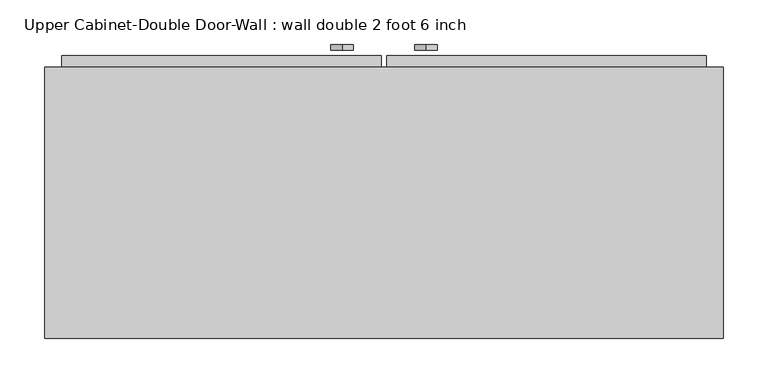
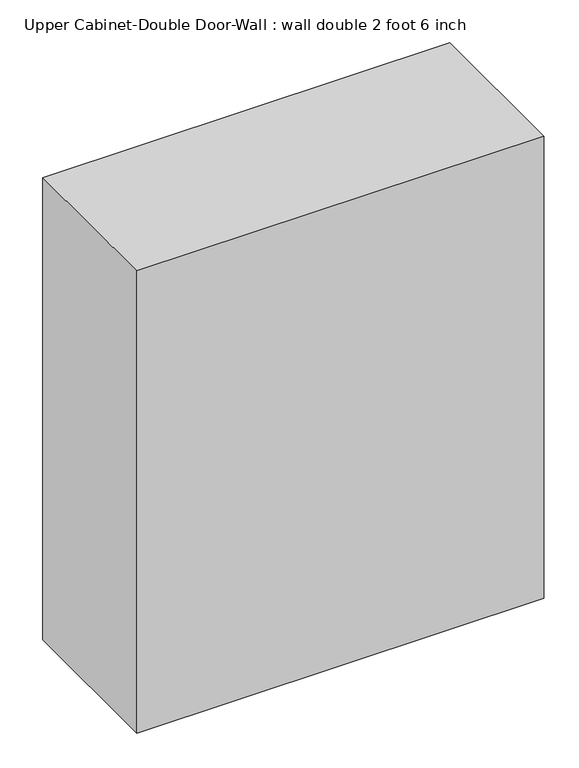
"""IFC4 building model written with IfcOpenShell, lengths in millimetres: furniture geometry, Upper Cabinet-Double Door-Wall : wall double 2 foot 6 inch."""

from ifc_helpers import new_model, si_unit, point, frame, frame_2d, origin, place, context, project, spatial, polyline, circle_curve, trimmed, segment, composite_curve, outline, extrude, faceted_brep, source, transform, mapped, element, save


def upper_cabinet_double_door_wall_wall_double_2_foot_6_inch_6202fb0c(model_context):
    return source(origin(), model_context, "Body", "SolidModel", [
        faceted_brep([(-351.2288372, 56.35625, 2133.6), (-351.2288372, 56.35625, 1219.2), (410.7711628, 56.35625, 1219.2), (410.7711628, 56.35625, 2133.6), (-351.2288372, 361.15625, 2133.6), (410.7711628, 361.15625, 2133.6), (410.7711628, 361.15625, 1219.2), (-351.2288372, 361.15625, 1219.2), (-332.1788372, 361.15625, 2114.55), (-332.1788372, 361.15625, 1238.25), (391.7211628, 361.15625, 1238.25), (391.7211628, 361.15625, 2114.55), (391.7211628, 75.40625, 2114.55), (-332.1788372, 75.40625, 2114.55), (391.7211628, 75.40625, 1238.25), (-332.1788372, 75.40625, 1238.25)], [[[0, 1, 2, 3]], [[4, 5, 6, 7], [8, 9, 10, 11]], [[1, 0, 4, 7]], [[2, 1, 7, 6]], [[3, 2, 6, 5]], [[0, 3, 5, 4]], [[8, 11, 12, 13]], [[11, 10, 14, 12]], [[10, 9, 15, 14]], [[9, 8, 13, 15]], [[13, 12, 14, 15]]]),
        extrude(outline(polyline([(32.9461628, 373.85625), (391.7211628, 373.85625), (391.7211628, 342.10625), (32.9461628, 342.10625), (32.9461628, 373.85625)])), frame((0.0, 0.0, 1238.25), z_axis=(0.0, 0.0, 1.0), x_axis=(1.0, 0.0, 0.0)), (0.0, 0.0, 1.0), 876.3),
        extrude(outline(polyline([(-332.1788372, 373.85625), (26.5961628, 373.85625), (26.5961628, 342.10625), (-332.1788372, 342.10625), (-332.1788372, 373.85625)])), frame((0.0, 0.0, 1238.25), z_axis=(0.0, 0.0, 1.0), x_axis=(1.0, 0.0, 0.0)), (0.0, 0.0, 1.0), 876.3),
        extrude(outline(composite_curve([segment(trimmed(circle_curve(frame_2d((1381.4214732, 76.8007051)), 12.7), [point((1368.7214732, 76.8007051))], [point((1394.1214732, 76.8007051))], False, "CARTESIAN"), True, "CONTINUOUS"), segment(trimmed(circle_curve(frame_2d((1381.4214732, 76.8007051)), 12.7), [point((1394.1214732, 76.8007051))], [point((1368.7214732, 76.8007051))], False, "CARTESIAN"), True, "CONTINUOUS")], self_intersect=False)), frame((0.0, 380.20625, 0.0), z_axis=(0.0, 1.0, 0.0), x_axis=(0.0, 0.0, 1.0)), (0.0, 0.0, 1.0), 6.35),
        extrude(outline(composite_curve([segment(trimmed(circle_curve(frame_2d((1381.4214732, -17.2583796)), 12.7), [point((1368.7214732, -17.2583796))], [point((1394.1214732, -17.2583796))], False, "CARTESIAN"), True, "CONTINUOUS"), segment(trimmed(circle_curve(frame_2d((1381.4214732, -17.2583796)), 12.7), [point((1394.1214732, -17.2583796))], [point((1368.7214732, -17.2583796))], False, "CARTESIAN"), True, "CONTINUOUS")], self_intersect=False)), frame((0.0, 380.20625, 0.0), z_axis=(0.0, 1.0, 0.0), x_axis=(0.0, 0.0, 1.0)), (0.0, 0.0, 1.0), 6.35),
    ])


if __name__ == "__main__":
    model = new_model("IFC4")
    model_context = context("Model", 3, world=origin())
    ifc_project = project(units=[si_unit("LENGTHUNIT", "METRE", prefix="MILLI")], contexts=[model_context])
    site = spatial("IfcSite", under=ifc_project)
    building = spatial("IfcBuilding", under=site)
    placement = place(None, origin())
    upper_cabinet_double_door_wall_wall_double_2_foot_6_inch_shape = upper_cabinet_double_door_wall_wall_double_2_foot_6_inch_6202fb0c(model_context)
    element("IfcFurniture", 1, ObjectType="Upper Cabinet-Double Door-Wall : wall double 2 foot 6 inch", at=placement, inside=building, context=model_context, shape_type="MappedRepresentation", body=[
        mapped(upper_cabinet_double_door_wall_wall_double_2_foot_6_inch_shape, transform((0.0, 0.0, 0.0), x_axis=(1.0, 0.0, 0.0), y_axis=(0.0, 1.0, 0.0), z_axis=(0.0, 0.0, 1.0))),
    ])
    save(model, "model.ifc")

# Revit data of these elements
# Type "Upper Cabinet-Double Door-Wall : wall double 2 foot 6 inch"
#   Assembly Code = "C1030410"
#   Depth = 1' - 0"
#   Height = 3' - 0"
#   Top Of Cabinet = 7' - 0"
#   Width = 2' - 6"
#   Cabinet Material = Base cabinet 2120100 Aspekt - 83012120100 - White
#   Door/Drawer Material = Base cabinet 2120100 Aspekt - 83012120100 - White
#   Handle Material = Cabinets - Handles
#   Default Elevation = 0
# Element 1 (IfcFurniture, "Upper Cabinet-Double Door-Wall : wall double 2 foot 6 inch")
#   Materials on its faces: "Base cabinet 2120100 Aspekt - 83012120100 - White"
# Materials
#   "Base cabinet 2120100 Aspekt - 83012120100 - White": class "Miscellaneous", colour RGB 255 255 255, transparency 0, Manufacturer = "Marbodal", URL = "http://www.marbodal.se", Cost = 0
#   "Cabinets - Handles": class "Metal", colour RGB 57 57 57, transparency 0
